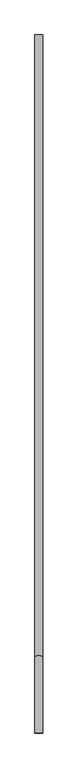
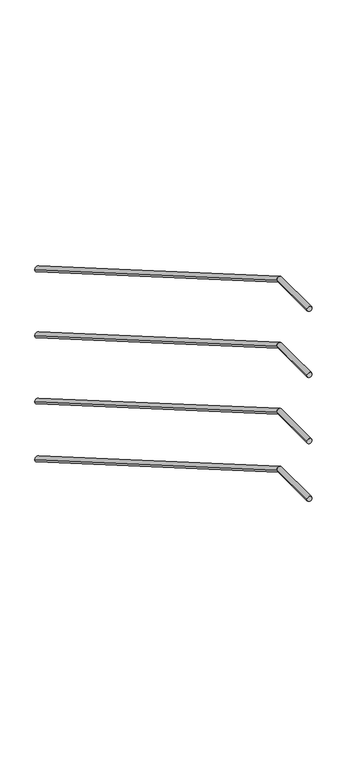
"""IFC4 building model written with IfcOpenShell, lengths in millimetres: railing geometry."""

from ifc_helpers import new_model, si_unit, frame, origin, place, context, project, spatial, circle_curve, ellipse_curve, source, transform, mapped, element, save
from ifc_brep_helpers import plane_surface, cylinder_surface, advanced_brep


def railing_4dfa4352(model_context):
    return source(origin(), model_context, "Body", "AdvancedBrep", [
        advanced_brep(
        [(-1709.6, 15799.5208589, 5689.6773196), (-1739.6, 15799.5208589, 5689.6773196), (-1709.6, 13395.4833005, 7084.9618634), (-1739.6, 13395.4833005, 7084.9618634), (-1709.6, 13099.5208589, 7084.9618634), (-1739.6, 13099.5208589, 7084.9618634)],
        [
            (0, 1, ellipse_curve(frame((-1724.6, 15799.5208589, 5689.6773196), z_axis=(0.0, 1.0, 0.0), x_axis=(0.0, 0.0, -1.0)), 17.3433672, 15.0)),
            (1, 0, ellipse_curve(frame((-1724.6, 15799.5208589, 5689.6773196), z_axis=(0.0, 1.0, 0.0), x_axis=(0.0, 0.0, -1.0)), 17.3433672, 15.0)),
            (0, 2),
            (2, 3, ellipse_curve(frame((-1724.6, 13395.4833005, 7084.9618634), z_axis=(0.0, 0.9656303515230847, -0.25991926480621574), x_axis=(0.0, -0.25991926480621586, -0.9656303515230849)), 15.5338945, 15.0)),
            (3, 1),
            (3, 2, ellipse_curve(frame((-1724.6, 13395.4833005, 7084.9618634), z_axis=(0.0, 0.9656303515230847, -0.25991926480621574), x_axis=(0.0, -0.25991926480621586, -0.9656303515230849)), 15.5338945, 15.0)),
            (4, 5, circle_curve(frame((-1724.6, 13099.5208589, 7084.9618634), z_axis=(0.0, -1.0, 0.0), x_axis=(-1.0, 0.0, 0.0)), 15.0)),
            (5, 4, circle_curve(frame((-1724.6, 13099.5208589, 7084.9618634), z_axis=(0.0, -1.0, 0.0), x_axis=(-1.0, 0.0, 0.0)), 15.0)),
            (2, 4),
            (5, 3),
        ],
        [
            plane_surface(frame((-1724.6, 15799.5208589, 5707.0206869), z_axis=(0.0, 1.0, 0.0), x_axis=(0.0, 0.0, -1.0))),
            cylinder_surface(frame((-1724.6, 15791.991281, 5694.0474276), z_axis=(0.0, 0.8648839515651926, -0.5019718620848959), x_axis=(-1.0, 0.0, 0.0)), 15.0),
            plane_surface(frame((-1724.6, 13099.5208589, 7099.9618634), z_axis=(0.0, -1.0, 0.0), x_axis=(0.0, 0.0, -1.0))),
            cylinder_surface(frame((-1724.6, 13399.5208589, 7084.9618634), z_axis=(0.0, 1.0, 0.0), x_axis=(-1.0, 0.0, 0.0)), 15.0),
        ],
        [
            (0, [[1, 2]]),
            (1, [[-1, 3, 4, 5]]),
            (1, [[-2, -5, 6, -3]]),
            (2, [[7, 8]]),
            (3, [[-4, 9, -8, 10]]),
            (3, [[-6, -10, -7, -9]]),
        ],
    ),
        advanced_brep(
        [(-1709.6, 15799.5208589, 4889.6773196), (-1739.6, 15799.5208589, 4889.6773196), (-1709.6, 13395.4833005, 6284.9618634), (-1739.6, 13395.4833005, 6284.9618634), (-1709.6, 13099.5208589, 6284.9618634), (-1739.6, 13099.5208589, 6284.9618634)],
        [
            (0, 1, ellipse_curve(frame((-1724.6, 15799.5208589, 4889.6773196), z_axis=(0.0, 1.0, 0.0), x_axis=(0.0, 0.0, -1.0)), 17.3433672, 15.0)),
            (1, 0, ellipse_curve(frame((-1724.6, 15799.5208589, 4889.6773196), z_axis=(0.0, 1.0, 0.0), x_axis=(0.0, 0.0, -1.0)), 17.3433672, 15.0)),
            (0, 2),
            (2, 3, ellipse_curve(frame((-1724.6, 13395.4833005, 6284.9618634), z_axis=(0.0, 0.9656303515230847, -0.25991926480621574), x_axis=(0.0, -0.25991926480621586, -0.9656303515230849)), 15.5338945, 15.0)),
            (3, 1),
            (3, 2, ellipse_curve(frame((-1724.6, 13395.4833005, 6284.9618634), z_axis=(0.0, 0.9656303515230847, -0.25991926480621574), x_axis=(0.0, -0.25991926480621586, -0.9656303515230849)), 15.5338945, 15.0)),
            (4, 5, circle_curve(frame((-1724.6, 13099.5208589, 6284.9618634), z_axis=(0.0, -1.0, 0.0), x_axis=(-1.0, 0.0, 0.0)), 15.0)),
            (5, 4, circle_curve(frame((-1724.6, 13099.5208589, 6284.9618634), z_axis=(0.0, -1.0, 0.0), x_axis=(-1.0, 0.0, 0.0)), 15.0)),
            (2, 4),
            (5, 3),
        ],
        [
            plane_surface(frame((-1724.6, 15799.5208589, 4907.0206869), z_axis=(0.0, 1.0, 0.0), x_axis=(0.0, 0.0, -1.0))),
            cylinder_surface(frame((-1724.6, 15791.991281, 4894.0474276), z_axis=(0.0, 0.8648839515651926, -0.5019718620848959), x_axis=(-1.0, 0.0, 0.0)), 15.0),
            plane_surface(frame((-1724.6, 13099.5208589, 6299.9618634), z_axis=(0.0, -1.0, 0.0), x_axis=(0.0, 0.0, -1.0))),
            cylinder_surface(frame((-1724.6, 13399.5208589, 6284.9618634), z_axis=(0.0, 1.0, 0.0), x_axis=(-1.0, 0.0, 0.0)), 15.0),
        ],
        [
            (0, [[1, 2]]),
            (1, [[-1, 3, 4, 5]]),
            (1, [[-2, -5, 6, -3]]),
            (2, [[7, 8]]),
            (3, [[-4, 9, -8, 10]]),
            (3, [[-6, -10, -7, -9]]),
        ],
    ),
        advanced_brep(
        [(-1709.6, 15799.5208589, 5289.6773196), (-1739.6, 15799.5208589, 5289.6773196), (-1709.6, 13395.4833005, 6684.9618634), (-1739.6, 13395.4833005, 6684.9618634), (-1709.6, 13099.5208589, 6684.9618634), (-1739.6, 13099.5208589, 6684.9618634)],
        [
            (0, 1, ellipse_curve(frame((-1724.6, 15799.5208589, 5289.6773196), z_axis=(0.0, 1.0, 0.0), x_axis=(0.0, 0.0, -1.0)), 17.3433672, 15.0)),
            (1, 0, ellipse_curve(frame((-1724.6, 15799.5208589, 5289.6773196), z_axis=(0.0, 1.0, 0.0), x_axis=(0.0, 0.0, -1.0)), 17.3433672, 15.0)),
            (0, 2),
            (2, 3, ellipse_curve(frame((-1724.6, 13395.4833005, 6684.9618634), z_axis=(0.0, 0.9656303515230847, -0.25991926480621574), x_axis=(0.0, -0.25991926480621586, -0.9656303515230849)), 15.5338945, 15.0)),
            (3, 1),
            (3, 2, ellipse_curve(frame((-1724.6, 13395.4833005, 6684.9618634), z_axis=(0.0, 0.9656303515230847, -0.25991926480621574), x_axis=(0.0, -0.25991926480621586, -0.9656303515230849)), 15.5338945, 15.0)),
            (4, 5, circle_curve(frame((-1724.6, 13099.5208589, 6684.9618634), z_axis=(0.0, -1.0, 0.0), x_axis=(-1.0, 0.0, 0.0)), 15.0)),
            (5, 4, circle_curve(frame((-1724.6, 13099.5208589, 6684.9618634), z_axis=(0.0, -1.0, 0.0), x_axis=(-1.0, 0.0, 0.0)), 15.0)),
            (2, 4),
            (5, 3),
        ],
        [
            plane_surface(frame((-1724.6, 15799.5208589, 5307.0206869), z_axis=(0.0, 1.0, 0.0), x_axis=(0.0, 0.0, -1.0))),
            cylinder_surface(frame((-1724.6, 15791.991281, 5294.0474276), z_axis=(0.0, 0.8648839515651926, -0.5019718620848959), x_axis=(-1.0, 0.0, 0.0)), 15.0),
            plane_surface(frame((-1724.6, 13099.5208589, 6699.9618634), z_axis=(0.0, -1.0, 0.0), x_axis=(0.0, 0.0, -1.0))),
            cylinder_surface(frame((-1724.6, 13399.5208589, 6684.9618634), z_axis=(0.0, 1.0, 0.0), x_axis=(-1.0, 0.0, 0.0)), 15.0),
        ],
        [
            (0, [[1, 2]]),
            (1, [[-1, 3, 4, 5]]),
            (1, [[-2, -5, 6, -3]]),
            (2, [[7, 8]]),
            (3, [[-4, 9, -8, 10]]),
            (3, [[-6, -10, -7, -9]]),
        ],
    ),
        advanced_brep(
        [(-1709.6, 15799.5208589, 4539.6773196), (-1739.6, 15799.5208589, 4539.6773196), (-1709.6, 13395.4833005, 5934.9618634), (-1739.6, 13395.4833005, 5934.9618634), (-1709.6, 13099.5208589, 5934.9618634), (-1739.6, 13099.5208589, 5934.9618634)],
        [
            (0, 1, ellipse_curve(frame((-1724.6, 15799.5208589, 4539.6773196), z_axis=(0.0, 1.0, 0.0), x_axis=(0.0, 0.0, -1.0)), 17.3433672, 15.0)),
            (1, 0, ellipse_curve(frame((-1724.6, 15799.5208589, 4539.6773196), z_axis=(0.0, 1.0, 0.0), x_axis=(0.0, 0.0, -1.0)), 17.3433672, 15.0)),
            (0, 2),
            (2, 3, ellipse_curve(frame((-1724.6, 13395.4833005, 5934.9618634), z_axis=(0.0, 0.9656303515230847, -0.25991926480621574), x_axis=(0.0, -0.25991926480621586, -0.9656303515230849)), 15.5338945, 15.0)),
            (3, 1),
            (3, 2, ellipse_curve(frame((-1724.6, 13395.4833005, 5934.9618634), z_axis=(0.0, 0.9656303515230847, -0.25991926480621574), x_axis=(0.0, -0.25991926480621586, -0.9656303515230849)), 15.5338945, 15.0)),
            (4, 5, circle_curve(frame((-1724.6, 13099.5208589, 5934.9618634), z_axis=(0.0, -1.0, 0.0), x_axis=(-1.0, 0.0, 0.0)), 15.0)),
            (5, 4, circle_curve(frame((-1724.6, 13099.5208589, 5934.9618634), z_axis=(0.0, -1.0, 0.0), x_axis=(-1.0, 0.0, 0.0)), 15.0)),
            (2, 4),
            (5, 3),
        ],
        [
            plane_surface(frame((-1724.6, 15799.5208589, 4557.0206869), z_axis=(0.0, 1.0, 0.0), x_axis=(0.0, 0.0, -1.0))),
            cylinder_surface(frame((-1724.6, 15791.991281, 4544.0474276), z_axis=(0.0, 0.8648839515651926, -0.5019718620848959), x_axis=(-1.0, 0.0, 0.0)), 15.0),
            plane_surface(frame((-1724.6, 13099.5208589, 5949.9618634), z_axis=(0.0, -1.0, 0.0), x_axis=(0.0, 0.0, -1.0))),
            cylinder_surface(frame((-1724.6, 13399.5208589, 5934.9618634), z_axis=(0.0, 1.0, 0.0), x_axis=(-1.0, 0.0, 0.0)), 15.0),
        ],
        [
            (0, [[1, 2]]),
            (1, [[-1, 3, 4, 5]]),
            (1, [[-2, -5, 6, -3]]),
            (2, [[7, 8]]),
            (3, [[-4, 9, -8, 10]]),
            (3, [[-6, -10, -7, -9]]),
        ],
    ),
    ])


if __name__ == "__main__":
    model = new_model("IFC4")
    model_context = context("Model", 3, world=origin())
    ifc_project = project(units=[si_unit("LENGTHUNIT", "METRE", prefix="MILLI")], contexts=[model_context])
    site = spatial("IfcSite", under=ifc_project)
    building = spatial("IfcBuilding", under=site)
    placement = place(None, origin())
    railing_shape = railing_4dfa4352(model_context)
    element("IfcRailing", 1, at=placement, inside=building, context=model_context, shape_type="MappedRepresentation", body=[
        mapped(railing_shape, transform((0.0, 0.0, 0.0), x_axis=(1.0, 0.0, 0.0), y_axis=(0.0, 1.0, 0.0), z_axis=(0.0, 0.0, 1.0))),
    ])
    save(model, "model.ifc")
